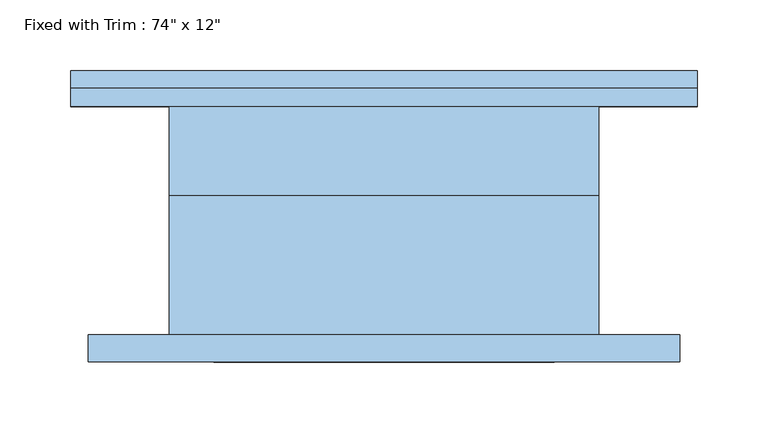
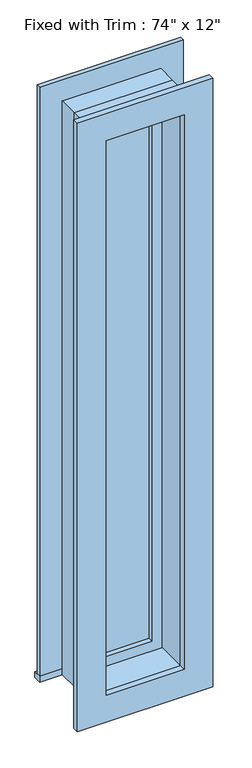
"""IFC4 building model written with IfcOpenShell, lengths in millimetres: window geometry."""

import ifcopenshell
import ifcopenshell.guid

model = None  # the IFC model being written
_history = None  # IfcOwnerHistory: only IFC2X3 demands one
_inside = {}  # id of a spatial element -> (the spatial element, [elements in it])
_under = {}  # id of a project, library or spatial element -> (it, [spatial elements below it])
_declared = {}  # id of a project -> (the project, [libraries it declares])
_typed = {}  # id of a type object -> (the type object, [elements of that type])
_made_of = {}  # id of a material, layer set ... -> (it, [elements and type objects made of it])


def new_model(schema):
    """Start an empty IFC model of exactly this schema.

    Asked for "IFC4X3", IfcOpenShell would pick the latest addendum, in which some entities
    have other attributes; the version numbers below select the first issue.
    IFC2X3 requires an IfcOwnerHistory on every rooted entity: one is made here for all.
    """
    global model, _history
    if schema == "IFC4X3":
        model = ifcopenshell.file(schema_version=(4, 3, 0, 0))
    else:
        model = ifcopenshell.file(schema=schema)
    _inside.clear()
    _under.clear()
    _declared.clear()
    _typed.clear()
    _made_of.clear()
    _history = None
    if model.schema == "IFC2X3":
        org = make("IfcOrganization", Name="unknown")
        user = make(
            "IfcPersonAndOrganization",
            ThePerson=make("IfcPerson", FamilyName="unknown"),
            TheOrganization=org,
        )
        app = make(
            "IfcApplication",
            ApplicationDeveloper=org,
            Version="unknown",
            ApplicationFullName="unknown",
            ApplicationIdentifier="unknown",
        )
        _history = make(
            "IfcOwnerHistory",
            OwningUser=user,
            OwningApplication=app,
            ChangeAction="ADDED",
            CreationDate=0,
        )
    return model


def make(cls, **values):
    """One entity of the class cls with the attributes given. An attribute that is None is left unset."""
    return model.create_entity(
        cls, **{name: value for name, value in values.items() if value is not None}
    )


def rooted(cls, **values):
    """An entity with a GlobalId (a new one), such as an element, a storey or a relation."""
    return make(cls, GlobalId=ifcopenshell.guid.new(), OwnerHistory=_history, **values)


def si_unit(unit_type, name, prefix=None):
    """IfcSIUnit, for example si_unit("LENGTHUNIT", "METRE", prefix="MILLI")."""
    return make("IfcSIUnit", UnitType=unit_type, Prefix=prefix, Name=name)


def assignment(units):
    """IfcUnitAssignment: the units of a project."""
    return None if units is None else make("IfcUnitAssignment", Units=units)


def point(xyz):
    """IfcCartesianPoint."""
    return None if xyz is None else make("IfcCartesianPoint", Coordinates=xyz)


def direction(xyz):
    """IfcDirection."""
    return None if xyz is None else make("IfcDirection", DirectionRatios=xyz)


def frame(location, z_axis=None, x_axis=None):
    """IfcAxis2Placement3D, a coordinate frame: its origin and axes. An axis left out is left unset."""
    return make(
        "IfcAxis2Placement3D",
        Location=point(location),
        Axis=direction(z_axis),
        RefDirection=direction(x_axis),
    )


def origin():
    """The frame at (0, 0, 0) with its axes left unset."""
    return frame((0.0, 0.0, 0.0))


def place(relative_to, where):
    """IfcLocalPlacement: puts the frame where relative to a parent placement (None: the world)."""
    return make(
        "IfcLocalPlacement", PlacementRelTo=relative_to, RelativePlacement=where
    )


def context(
    kind, dimensions, precision=None, world=None, true_north=None, identifier=None
):
    """IfcGeometricRepresentationContext, for example the 3D "Model" context."""
    return make(
        "IfcGeometricRepresentationContext",
        ContextIdentifier=identifier,
        ContextType=kind,
        CoordinateSpaceDimension=dimensions,
        Precision=precision,
        WorldCoordinateSystem=world,
        TrueNorth=true_north,
    )


def project(units=None, contexts=None):
    """IfcProject with its units and contexts."""
    return rooted(
        "IfcProject",
        Name="project",
        RepresentationContexts=contexts,
        UnitsInContext=assignment(units),
    )


def spatial(cls, under=None, at=None, **own):
    """A site, building, storey or space (cls), placed at a placement, below another one or the project."""
    s = rooted(cls, ObjectPlacement=at, **own)
    if under is not None:
        _under.setdefault(under.id(), (under, []))[1].append(s)
    return s


def polyline(points):
    """IfcPolyline through the points."""
    return make("IfcPolyline", Points=[point(p) for p in points])


def outline(outer, holes=None, kind="AREA"):
    """IfcArbitraryClosedProfileDef: a profile drawn as a closed curve; with holes, ...WithVoids."""
    if holes is None:
        return make("IfcArbitraryClosedProfileDef", ProfileType=kind, OuterCurve=outer)
    return make(
        "IfcArbitraryProfileDefWithVoids",
        ProfileType=kind,
        OuterCurve=outer,
        InnerCurves=holes,
    )


def extrude(swept, where, along, depth):
    """IfcExtrudedAreaSolid: the profile swept, set in the frame where, extruded along a direction by depth."""
    return make(
        "IfcExtrudedAreaSolid",
        SweptArea=swept,
        Position=where,
        ExtrudedDirection=direction(along),
        Depth=depth,
    )


def shape(context_of_items, identifier, shape_type, items):
    """IfcShapeRepresentation: the items that make up one representation, for example the "Body"."""
    return make(
        "IfcShapeRepresentation",
        ContextOfItems=context_of_items,
        RepresentationIdentifier=identifier,
        RepresentationType=shape_type,
        Items=items,
    )


def source(mapping_origin, context_of_items, identifier, shape_type, items):
    """IfcRepresentationMap: a shape defined once, which mapped items show again and again."""
    return make(
        "IfcRepresentationMap",
        MappingOrigin=mapping_origin,
        MappedRepresentation=shape(context_of_items, identifier, shape_type, items),
    )


def transform(
    local_origin,
    x_axis=None,
    y_axis=None,
    z_axis=None,
    scale=None,
    scale2=None,
    scale3=None,
    uniform=True,
):
    """IfcCartesianTransformationOperator3D, or its non-uniform kind. x_axis, y_axis, z_axis: its Axis1, 2, 3."""
    if uniform:
        return make(
            "IfcCartesianTransformationOperator3D",
            Axis1=direction(x_axis),
            Axis2=direction(y_axis),
            LocalOrigin=point(local_origin),
            Scale=scale,
            Axis3=direction(z_axis),
        )
    return make(
        "IfcCartesianTransformationOperator3DnonUniform",
        Axis1=direction(x_axis),
        Axis2=direction(y_axis),
        LocalOrigin=point(local_origin),
        Scale=scale,
        Axis3=direction(z_axis),
        Scale2=scale2,
        Scale3=scale3,
    )


def mapped(mapping_source, mapping_target):
    """IfcMappedItem: shows the shape of a source again, moved by a transform."""
    return make(
        "IfcMappedItem", MappingSource=mapping_source, MappingTarget=mapping_target
    )


def made_of(thing, what):
    """Note that an element or type object is made of a material, layer set ...; save() writes the relation."""
    if what is not None:
        _made_of.setdefault(what.id(), (what, []))[1].append(thing)
    return thing


def element(
    cls,
    number,
    at=None,
    inside=None,
    cuts=None,
    type_object=None,
    material=None,
    context=None,
    identifier="Body",
    shape_type=None,
    held_by="IfcProductDefinitionShape",
    body=None,
    shapes=None,
    **own,
):
    """One element of the class cls, such as IfcWall. Its Tag is "e" and its number.

    at: its placement. inside: the storey or other place that contains it. cuts: it is an
    opening in that element (IfcRelVoidsElement). A single representation is given by context,
    identifier, shape_type and body (its items); several are given by shapes. held_by: the class
    of the entity that holds the representations. save() writes the other relations.
    """
    e = rooted(cls, Tag="e%d" % number, ObjectPlacement=at, **own)
    if body is not None:
        shapes = [shape(context, identifier, shape_type, body)]
    if shapes is not None:
        e.Representation = make(held_by, Representations=shapes)
    if inside is not None:
        _inside.setdefault(inside.id(), (inside, []))[1].append(e)
    if cuts is not None:
        rooted(
            "IfcRelVoidsElement", RelatingBuildingElement=cuts, RelatedOpeningElement=e
        )
    if type_object is not None:
        _typed.setdefault(type_object.id(), (type_object, []))[1].append(e)
    return made_of(e, material)


def aggregate(whole, parts):
    """IfcRelAggregates: a whole, such as a stair, and the parts it consists of."""
    return rooted("IfcRelAggregates", RelatingObject=whole, RelatedObjects=parts)


def save(model, path):
    """Write the relations noted so far, then the file.

    IfcRelAggregates (storeys below a building ...), IfcRelContainedInSpatialStructure (elements
    in a storey), IfcRelDefinesByType, IfcRelAssociatesMaterial and IfcRelDeclares: one each for
    every whole, place, type object, material and project.
    """
    for whole, parts in _under.values():
        aggregate(whole, parts)
    for where, things in _inside.values():
        rooted(
            "IfcRelContainedInSpatialStructure",
            RelatedElements=things,
            RelatingStructure=where,
        )
    for kind, things in _typed.values():
        rooted("IfcRelDefinesByType", RelatedObjects=things, RelatingType=kind)
    for what, things in _made_of.values():
        rooted("IfcRelAssociatesMaterial", RelatedObjects=things, RelatingMaterial=what)
    for by, libraries in _declared.values():
        rooted("IfcRelDeclares", RelatingContext=by, RelatedDefinitions=libraries)
    model.write(path)


def window_a6f95507(model_context):
    return source(origin(), model_context, "Body", "SweptSolid", [
        extrude(outline(polyline([(-260.35, 106.3625), (184.15, 106.3625), (184.15, 80.9625), (-260.35, 80.9625), (-260.35, 106.3625)])), frame((0.0, 0.0, 914.4), z_axis=(0.0, 0.0, 1.0), x_axis=(1.0, 0.0, 0.0)), (0.0, 0.0, 1.0), 19.05),
        extrude(outline(polyline([(2774.95, -171.45), (2774.95, 95.25), (933.45, 95.25), (933.45, 184.15), (2863.85, 184.15), (2863.85, -260.35), (933.45, -260.35), (933.45, -171.45), (2774.95, -171.45)])), frame((0.0, 80.9625, 0.0), z_axis=(0.0, 1.0, 0.0), x_axis=(0.0, 0.0, 1.0)), (0.0, 0.0, 1.0), 12.7),
        extrude(outline(polyline([(2851.15, 171.45), (2851.15, -247.65), (857.25, -247.65), (857.25, 171.45), (2851.15, 171.45)]), holes=[polyline([(2762.25, 82.55), (946.15, 82.55), (946.15, -158.75), (2762.25, -158.75), (2762.25, 82.55)])]), frame((0.0, -100.0125, 0.0), z_axis=(0.0, 1.0, 0.0), x_axis=(0.0, 0.0, 1.0)), (0.0, 0.0, 1.0), 19.05),
        extrude(outline(polyline([(50.8, 33.3375), (-127.0, 33.3375), (-127.0, 46.0375), (50.8, 46.0375), (50.8, 33.3375)])), frame((0.0, 0.0, 977.9), z_axis=(0.0, 0.0, 1.0), x_axis=(1.0, 0.0, 0.0)), (0.0, 0.0, 1.0), 1752.6),
        extrude(outline(polyline([(2774.95, -171.45), (933.45, -171.45), (933.45, 95.25), (2774.95, 95.25), (2774.95, -171.45)]), holes=[polyline([(2730.5, -127.0), (2730.5, 50.8), (977.9, 50.8), (977.9, -127.0), (2730.5, -127.0)])]), frame((0.0, 17.4625, 0.0), z_axis=(0.0, 1.0, 0.0), x_axis=(0.0, 0.0, 1.0)), (0.0, 0.0, 1.0), 44.45),
        extrude(outline(polyline([(2794.0, -190.5), (914.4, -190.5), (914.4, 114.3), (2794.0, 114.3), (2794.0, -190.5)]), holes=[polyline([(2762.25, -158.75), (2762.25, 82.55), (946.15, 82.55), (946.15, -158.75), (2762.25, -158.75)])]), frame((0.0, -80.9625, 0.0), z_axis=(0.0, 1.0, 0.0), x_axis=(0.0, 0.0, 1.0)), (0.0, 0.0, 1.0), 98.425),
        extrude(outline(polyline([(2794.0, 114.3), (2794.0, -190.5), (914.4, -190.5), (914.4, 114.3), (2794.0, 114.3)]), holes=[polyline([(2774.95, 95.25), (933.45, 95.25), (933.45, -171.45), (2774.95, -171.45), (2774.95, 95.25)])]), frame((0.0, 17.4625, 0.0), z_axis=(0.0, 1.0, 0.0), x_axis=(0.0, 0.0, 1.0)), (0.0, 0.0, 1.0), 63.5),
    ])


if __name__ == "__main__":
    model = new_model("IFC4")
    model_context = context("Model", 3, world=origin())
    ifc_project = project(units=[si_unit("LENGTHUNIT", "METRE", prefix="MILLI")], contexts=[model_context])
    site = spatial("IfcSite", under=ifc_project)
    building = spatial("IfcBuilding", under=site)
    placement = place(None, origin())
    window_shape = window_a6f95507(model_context)
    element("IfcWindow", 1, ObjectType="Fixed with Trim : 74\" x 12\"", at=placement, inside=building, context=model_context, shape_type="MappedRepresentation", body=[
        mapped(window_shape, transform((0.0, 0.0, 0.0), x_axis=(1.0, 0.0, 0.0), y_axis=(0.0, 1.0, 0.0), z_axis=(0.0, 0.0, 1.0))),
    ])
    save(model, "model.ifc")

# Revit data of these elements
# Type "Fixed with Trim : 74\" x 12\""
#   Type Mark = "60"
#   COBie.Type.CreatedBy = "doug.wood@us.ibm.com"
#   COBie.Type.CreatedOn = "2016-04-14T02:07:26"
#   COBie.Type.Name = "Windows_Fixed with Trim_74\" x 12\"_60"
#   COBie.Type.Category = "23-30 20 17 11 : Fixed Windows"
#   COBie.Type.Description = "Fixed with Trim_74\" x 12\""
#   COBie.Type.Manufacturer = ""
#   COBie.Type.ModelNumber = ""
#   Construction Type Id = "GSP4R"
#   Assembly Code = "B2020100"
#   Analytic Construction = "1/8 in Pilkington single glazing"
#   COBie.Type.ReplacementCost = 0
#   Visual Light Transmittance = 0.9
#   Solar Heat Gain Coefficient = 0.78
#   Heat Transfer Coefficient (U) = 3.6886 W/(m²·K)
#   Height = 6' - 2"
#   Default Sill Height = 3' - 0"
#   Trim Projection - Ext. = 0' - 0 1/2"
#   Trim Projection - Int. = 0' - 0 3/4"
#   Trim Width - Exterior = 0' - 3 1/2"
#   Trim Width - Interior = 0' - 3 1/2"
#   Width = 1' - 0"
#   Window Inset = 0' - 0 3/4"
#   COBie.Type = no
#   Glass Pane Material = Glass
#   Sash Material = Sash - White
#   Trim Exterior Material = Trim - White
#   Trim Interior Material = Trim - White
#   Wall Closure = (empty or 0)
# Element 1 (IfcWindow, "Fixed with Trim : 74\" x 12\"")
#   Materials on its faces: "Sash - White", "Trim - White", "Glass"
# Materials
#   "Glass": class "Glass", colour RGB 0 128 192, transparency 0.75, Description = "Soda Lime Glass", Cost = 0
#   "Sash - White": class "Wood", colour RGB 255 255 255, transparency 0, Cost = 0
#   "Trim - White": class "Wood", colour RGB 255 255 255, transparency 0, Cost = 0
